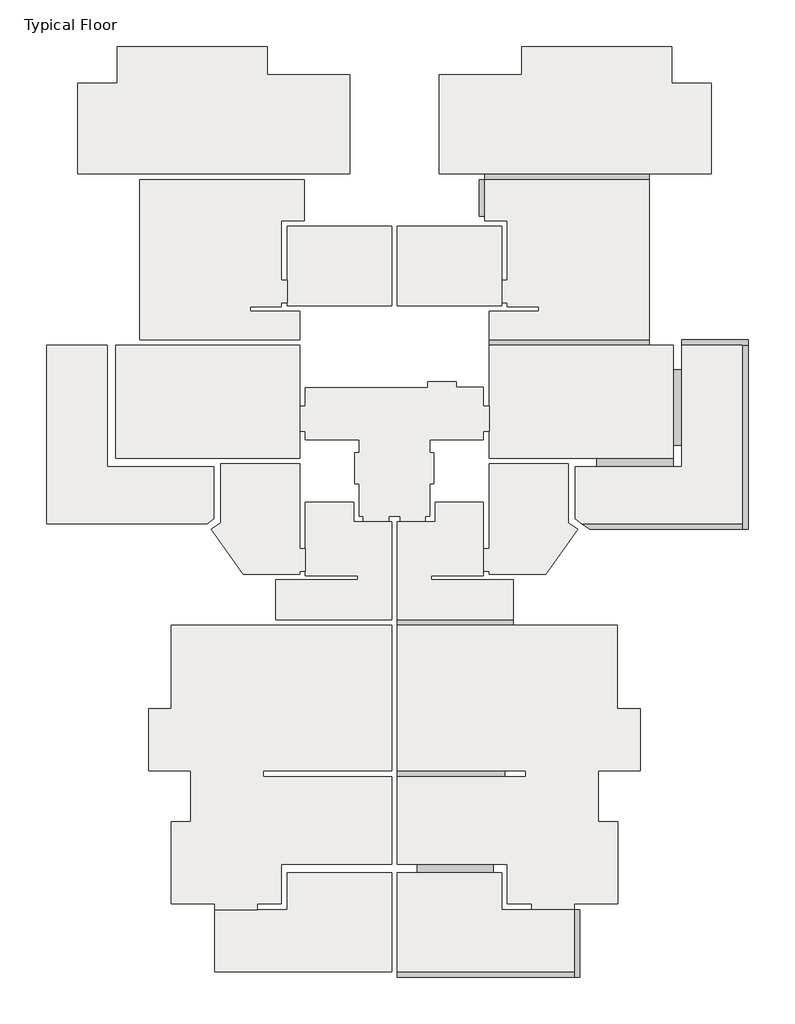
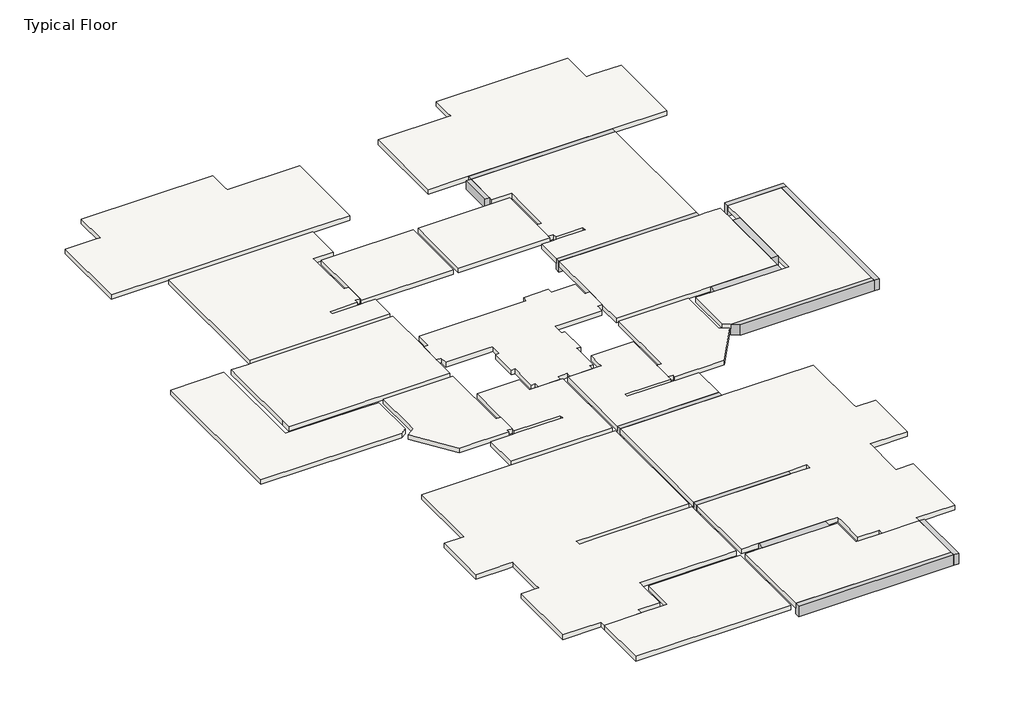
# One storey: 19 slabs, 13 beams.
"""IFC4 building model written with IfcOpenShell, lengths in millimetres."""

import ifcopenshell
import ifcopenshell.guid

model = None  # the IFC model being written
_history = None  # IfcOwnerHistory: only IFC2X3 demands one
_inside = {}  # id of a spatial element -> (the spatial element, [elements in it])
_under = {}  # id of a project, library or spatial element -> (it, [spatial elements below it])
_declared = {}  # id of a project -> (the project, [libraries it declares])
_typed = {}  # id of a type object -> (the type object, [elements of that type])
_made_of = {}  # id of a material, layer set ... -> (it, [elements and type objects made of it])


def new_model(schema):
    """Start an empty IFC model of exactly this schema.

    Asked for "IFC4X3", IfcOpenShell would pick the latest addendum, in which some entities
    have other attributes; the version numbers below select the first issue.
    IFC2X3 requires an IfcOwnerHistory on every rooted entity: one is made here for all.
    """
    global model, _history
    if schema == "IFC4X3":
        model = ifcopenshell.file(schema_version=(4, 3, 0, 0))
    else:
        model = ifcopenshell.file(schema=schema)
    _inside.clear()
    _under.clear()
    _declared.clear()
    _typed.clear()
    _made_of.clear()
    _history = None
    if model.schema == "IFC2X3":
        org = make("IfcOrganization", Name="unknown")
        user = make(
            "IfcPersonAndOrganization",
            ThePerson=make("IfcPerson", FamilyName="unknown"),
            TheOrganization=org,
        )
        app = make(
            "IfcApplication",
            ApplicationDeveloper=org,
            Version="unknown",
            ApplicationFullName="unknown",
            ApplicationIdentifier="unknown",
        )
        _history = make(
            "IfcOwnerHistory",
            OwningUser=user,
            OwningApplication=app,
            ChangeAction="ADDED",
            CreationDate=0,
        )
    return model


def make(cls, **values):
    """One entity of the class cls with the attributes given. An attribute that is None is left unset."""
    return model.create_entity(
        cls, **{name: value for name, value in values.items() if value is not None}
    )


def rooted(cls, **values):
    """An entity with a GlobalId (a new one), such as an element, a storey or a relation."""
    return make(cls, GlobalId=ifcopenshell.guid.new(), OwnerHistory=_history, **values)


def si_unit(unit_type, name, prefix=None):
    """IfcSIUnit, for example si_unit("LENGTHUNIT", "METRE", prefix="MILLI")."""
    return make("IfcSIUnit", UnitType=unit_type, Prefix=prefix, Name=name)


def assignment(units):
    """IfcUnitAssignment: the units of a project."""
    return None if units is None else make("IfcUnitAssignment", Units=units)


def point(xyz):
    """IfcCartesianPoint."""
    return None if xyz is None else make("IfcCartesianPoint", Coordinates=xyz)


def direction(xyz):
    """IfcDirection."""
    return None if xyz is None else make("IfcDirection", DirectionRatios=xyz)


def frame(location, z_axis=None, x_axis=None):
    """IfcAxis2Placement3D, a coordinate frame: its origin and axes. An axis left out is left unset."""
    return make(
        "IfcAxis2Placement3D",
        Location=point(location),
        Axis=direction(z_axis),
        RefDirection=direction(x_axis),
    )


def origin():
    """The frame at (0, 0, 0) with its axes left unset."""
    return frame((0.0, 0.0, 0.0))


def place(relative_to, where):
    """IfcLocalPlacement: puts the frame where relative to a parent placement (None: the world)."""
    return make(
        "IfcLocalPlacement", PlacementRelTo=relative_to, RelativePlacement=where
    )


def context(
    kind, dimensions, precision=None, world=None, true_north=None, identifier=None
):
    """IfcGeometricRepresentationContext, for example the 3D "Model" context."""
    return make(
        "IfcGeometricRepresentationContext",
        ContextIdentifier=identifier,
        ContextType=kind,
        CoordinateSpaceDimension=dimensions,
        Precision=precision,
        WorldCoordinateSystem=world,
        TrueNorth=true_north,
    )


def project(units=None, contexts=None):
    """IfcProject with its units and contexts."""
    return rooted(
        "IfcProject",
        Name="project",
        RepresentationContexts=contexts,
        UnitsInContext=assignment(units),
    )


def spatial(cls, under=None, at=None, **own):
    """A site, building, storey or space (cls), placed at a placement, below another one or the project."""
    s = rooted(cls, ObjectPlacement=at, **own)
    if under is not None:
        _under.setdefault(under.id(), (under, []))[1].append(s)
    return s


def faces_of(points, faces, orient=None, outer=None):
    """IfcFace entities. A face is a list of loops; a loop is a list of indices into points, from 0.

    orient and outer hold one flag for each loop. By default every Orientation is true, the
    first loop of a face is its IfcFaceOuterBound and the others are IfcFaceBound.
    """
    made = []
    for i, loops in enumerate(faces):
        bounds = []
        for j, loop in enumerate(loops):
            is_outer = j == 0 if outer is None else outer[i][j]
            bounds.append(
                make(
                    "IfcFaceOuterBound" if is_outer else "IfcFaceBound",
                    Bound=make("IfcPolyLoop", Polygon=[points[k] for k in loop]),
                    Orientation=True if orient is None else orient[i][j],
                )
            )
        made.append(make("IfcFace", Bounds=bounds))
    return made


def faceted_brep(points, faces, orient=None, outer=None, voids=None):
    """IfcFacetedBrep: a solid bounded by flat faces; with voids (closed shells), ...WithVoids."""
    shared = [point(p) for p in points]
    hull = make("IfcClosedShell", CfsFaces=faces_of(shared, faces, orient, outer))
    if voids is None:
        return make("IfcFacetedBrep", Outer=hull)
    return make(
        "IfcFacetedBrepWithVoids",
        Outer=hull,
        Voids=[
            make(cls, CfsFaces=faces_of(shared, fs, o, b)) for cls, fs, o, b in voids
        ],
    )


def shape(context_of_items, identifier, shape_type, items):
    """IfcShapeRepresentation: the items that make up one representation, for example the "Body"."""
    return make(
        "IfcShapeRepresentation",
        ContextOfItems=context_of_items,
        RepresentationIdentifier=identifier,
        RepresentationType=shape_type,
        Items=items,
    )


def made_of(thing, what):
    """Note that an element or type object is made of a material, layer set ...; save() writes the relation."""
    if what is not None:
        _made_of.setdefault(what.id(), (what, []))[1].append(thing)
    return thing


def element(
    cls,
    number,
    at=None,
    inside=None,
    cuts=None,
    type_object=None,
    material=None,
    context=None,
    identifier="Body",
    shape_type=None,
    held_by="IfcProductDefinitionShape",
    body=None,
    shapes=None,
    **own,
):
    """One element of the class cls, such as IfcWall. Its Tag is "e" and its number.

    at: its placement. inside: the storey or other place that contains it. cuts: it is an
    opening in that element (IfcRelVoidsElement). A single representation is given by context,
    identifier, shape_type and body (its items); several are given by shapes. held_by: the class
    of the entity that holds the representations. save() writes the other relations.
    """
    e = rooted(cls, Tag="e%d" % number, ObjectPlacement=at, **own)
    if body is not None:
        shapes = [shape(context, identifier, shape_type, body)]
    if shapes is not None:
        e.Representation = make(held_by, Representations=shapes)
    if inside is not None:
        _inside.setdefault(inside.id(), (inside, []))[1].append(e)
    if cuts is not None:
        rooted(
            "IfcRelVoidsElement", RelatingBuildingElement=cuts, RelatedOpeningElement=e
        )
    if type_object is not None:
        _typed.setdefault(type_object.id(), (type_object, []))[1].append(e)
    return made_of(e, material)


def aggregate(whole, parts):
    """IfcRelAggregates: a whole, such as a stair, and the parts it consists of."""
    return rooted("IfcRelAggregates", RelatingObject=whole, RelatedObjects=parts)


def save(model, path):
    """Write the relations noted so far, then the file.

    IfcRelAggregates (storeys below a building ...), IfcRelContainedInSpatialStructure (elements
    in a storey), IfcRelDefinesByType, IfcRelAssociatesMaterial and IfcRelDeclares: one each for
    every whole, place, type object, material and project.
    """
    for whole, parts in _under.values():
        aggregate(whole, parts)
    for where, things in _inside.values():
        rooted(
            "IfcRelContainedInSpatialStructure",
            RelatedElements=things,
            RelatingStructure=where,
        )
    for kind, things in _typed.values():
        rooted("IfcRelDefinesByType", RelatedObjects=things, RelatingType=kind)
    for what, things in _made_of.values():
        rooted("IfcRelAssociatesMaterial", RelatedObjects=things, RelatingMaterial=what)
    for by, libraries in _declared.values():
        rooted("IfcRelDeclares", RelatingContext=by, RelatedDefinitions=libraries)
    model.write(path)


model = new_model("IFC4")

# Units and contexts
model_context = context("Model", 3, world=origin())
ifc_project = project(units=[si_unit("LENGTHUNIT", "METRE", prefix="MILLI")], contexts=[model_context])

# Site, building, storey
site = spatial("IfcSite", under=ifc_project)
building = spatial("IfcBuilding", under=site)
storey = spatial("IfcBuildingStorey", under=building, Name="Typical Floor", Elevation=3000.0)

# Beams
placement = place(None, origin())
element("IfcBeam", 1, ObjectType="Concrete Rectengular Beam : 20/35", at=placement, inside=storey, context=model_context, shape_type="Brep", body=[
    faceted_brep([(7220.2839923, 5707.9881624, 3000.0), (7020.2839923, 5707.9881624, 3000.0), (7020.2839923, 4410.637169, 3000.0), (7220.2839923, 4410.637169, 3000.0), (7220.2839923, 5707.9881624, 2650.0), (7220.2839923, 5707.9881624, 2800.0), (7220.2839923, 4410.637169, 2650.0), (7020.2839923, 5707.9881624, 2650.0), (7020.2839923, 4410.637169, 2650.0)], [[[0, 1, 2, 3]], [[4, 5, 0, 3, 6]], [[7, 4, 6, 8]], [[1, 7, 8, 2]], [[1, 0, 5, 4, 7]], [[3, 2, 8, 6]]]),
])
element("IfcBeam", 2, ObjectType="Concrete Rectengular Beam : 20/45", at=placement, inside=storey, context=model_context, shape_type="Brep", body=[
    faceted_brep([(13024.2575022, -153.3363409, 3000.0), (13024.2575022, 46.6636591, 3000.0), (7369.9528665, 46.6636591, 3000.0), (7369.9528665, -153.3363409, 3000.0), (13024.2575022, -153.3363409, 2550.0), (7369.9528665, -153.3363409, 2800.0), (7369.9528665, -153.3363409, 2550.0), (13024.2575022, 46.6636591, 2550.0), (7369.9528665, 46.6636591, 2550.0), (13024.2575022, 46.6636591, 2800.0), (7369.9528665, 46.6636591, 2800.0)], [[[0, 1, 2, 3]], [[4, 0, 3, 5, 6]], [[7, 4, 6, 8]], [[1, 9, 7, 8, 10, 2]], [[1, 0, 4, 7, 9]], [[3, 2, 10, 8, 6, 5]]]),
])
element("IfcBeam", 3, ObjectType="Concrete Rectengular Beam : 20/45", at=placement, inside=storey, context=model_context, shape_type="Brep", body=[
    faceted_brep([(16525.1499872, -153.3363409, 3000.0), (16525.1499872, 46.6636591, 3000.0), (14175.1499872, 46.6636591, 3000.0), (14175.1499872, -153.3363409, 3000.0), (16325.1499872, -153.3363409, 3000.0), (16525.1499872, 46.6636591, 2550.0), (14175.1499872, 46.6636591, 2550.0), (16525.1499872, -153.3363409, 2550.0), (16325.1499872, -153.3363409, 2550.0), (14175.1499872, -153.3363409, 2550.0), (14175.1499872, -153.3363409, 2800.0)], [[[0, 1, 2, 3, 4]], [[1, 5, 6, 2]], [[5, 7, 8, 9, 6]], [[7, 0, 4, 3, 10, 9, 8]], [[3, 2, 6, 9, 10]], [[1, 0, 7, 5]]]),
])
element("IfcBeam", 4, ObjectType="Concrete Rectengular Beam : 20/45", at=placement, inside=storey, context=model_context, shape_type="Brep", body=[
    faceted_brep([(16325.1499872, -6653.3363409, 3000.0), (16525.1499872, -6653.3363409, 3000.0), (16525.1499872, -153.3363409, 3000.0), (16325.1499872, -153.3363409, 3000.0), (16325.1499872, -6453.3363409, 3000.0), (16525.1499872, -6653.3363409, 2550.0), (16525.1499872, -153.3363409, 2550.0), (16325.1499872, -6653.3363409, 2550.0), (16325.1499872, -6453.3363409, 2550.0), (16325.1499872, -153.3363409, 2550.0), (16325.1499872, -153.3363409, 2800.0)], [[[0, 1, 2, 3, 4]], [[1, 5, 6, 2]], [[5, 7, 8, 9, 6]], [[7, 0, 4, 3, 10, 9, 8]], [[3, 2, 6, 9, 10]], [[1, 0, 7, 5]]]),
])
element("IfcBeam", 5, ObjectType="Concrete Rectengular Beam : 20/45", at=placement, inside=storey, context=model_context, shape_type="Brep", body=[
    faceted_brep([(10651.3091706, -6453.3363409, 3000.0), (10931.7636873, -6652.8905163, 3000.0), (10931.4469171, -6653.3363409, 3000.0), (16325.1499872, -6653.3363409, 3000.0), (16325.1499872, -6453.3363409, 3000.0), (10931.4469171, -6653.3363409, 2550.0), (16325.1499872, -6653.3363409, 2550.0), (10931.7636873, -6652.8905163, 2550.0), (10651.3091706, -6453.3363409, 2550.0), (16325.1499872, -6453.3363409, 2550.0), (10651.3091706, -6453.3363409, 2800.0), (16325.1499872, -6453.3363409, 2800.0)], [[[0, 1, 2, 3, 4]], [[2, 5, 6, 3]], [[7, 8, 9, 6, 5]], [[8, 10, 0, 4, 11, 9]], [[1, 0, 10, 8, 7]], [[2, 1, 7, 5]], [[4, 3, 6, 9, 11]]]),
])
element("IfcBeam", 6, ObjectType="Concrete Rectengular Beam : 20/45", at=placement, inside=storey, context=model_context, shape_type="Brep", body=[
    faceted_brep([(10372.2707473, -22500.6211091, 3000.0), (10572.2707473, -22500.6211091, 3000.0), (10572.2707473, -20100.6211091, 3000.0), (10372.2707473, -20100.6211091, 3000.0), (10372.2707473, -22300.6211091, 3000.0), (10572.2707473, -22500.6211091, 2550.0), (10572.2707473, -20100.6211091, 2550.0), (10372.2707473, -22500.6211091, 2550.0), (10372.2707473, -22300.6211091, 2550.0), (10372.2707473, -20100.6211091, 2550.0), (10372.2707473, -20100.6211091, 2800.0)], [[[0, 1, 2, 3, 4]], [[1, 5, 6, 2]], [[5, 7, 8, 9, 6]], [[7, 0, 4, 3, 10, 9, 8]], [[3, 2, 6, 9, 10]], [[1, 0, 7, 5]]]),
])
element("IfcBeam", 7, ObjectType="Concrete Rectengular Beam : 20/45", at=placement, inside=storey, context=model_context, shape_type="Brep", body=[
    faceted_brep([(10372.2707473, -22500.6211091, 3000.0), (10372.2707473, -22300.6211091, 3000.0), (4123.5952506, -22300.6211091, 3000.0), (4123.5952506, -22500.6211091, 3000.0), (10372.2707473, -22500.6211091, 2550.0), (4123.5952506, -22500.6211091, 2550.0), (10372.2707473, -22300.6211091, 2550.0), (4123.5952506, -22300.6211091, 2550.0), (10372.2707473, -22300.6211091, 2800.0), (4123.5952506, -22300.6211091, 2800.0)], [[[0, 1, 2, 3]], [[4, 0, 3, 5]], [[6, 4, 5, 7]], [[1, 8, 6, 7, 9, 2]], [[1, 0, 4, 6, 8]], [[3, 2, 9, 7, 5]]]),
])
element("IfcBeam", 8, ObjectType="Concrete Rectengular Beam : 20/45", at=placement, inside=storey, context=model_context, shape_type="Brep", body=[
    faceted_brep([(7917.6091941, -15399.2157792, 3000.0), (7917.6091941, -15199.2157792, 3000.0), (4123.5952506, -15199.2157792, 3000.0), (4123.5952506, -15399.2157792, 3000.0), (7917.6091941, -15399.2157792, 2550.0), (7917.6091941, -15399.2157792, 2800.0), (4123.5952506, -15399.2157792, 2800.0), (4123.5952506, -15399.2157792, 2550.0), (7917.6091941, -15199.2157792, 2550.0), (4123.5952506, -15199.2157792, 2550.0), (7917.6091941, -15199.2157792, 2800.0), (4123.5952506, -15199.2157792, 2800.0)], [[[0, 1, 2, 3]], [[4, 5, 0, 3, 6, 7]], [[8, 4, 7, 9]], [[1, 10, 8, 9, 11, 2]], [[1, 0, 5, 4, 8, 10]], [[3, 2, 11, 9, 7, 6]]]),
])
element("IfcBeam", 9, ObjectType="Concrete Rectengular Beam : 20/45", at=placement, inside=storey, context=model_context, shape_type="Brep", body=[
    faceted_brep([(8220.6151181, -10045.6542217, 3000.0), (8220.6151181, -9845.6542217, 3000.0), (4123.5952506, -9845.6542217, 3000.0), (4123.5952506, -10045.6542217, 3000.0), (8220.6151181, -10045.6542217, 2550.0), (4123.5952506, -10045.6542217, 2800.0), (4123.5952506, -10045.6542217, 2550.0), (8220.6151181, -9845.6542217, 2550.0), (4123.5952506, -9845.6542217, 2550.0), (8220.6151181, -9845.6542217, 2800.0), (4123.5952506, -9845.6542217, 2800.0)], [[[0, 1, 2, 3]], [[4, 0, 3, 5, 6]], [[7, 4, 6, 8]], [[1, 9, 7, 8, 10, 2]], [[1, 0, 4, 7, 9]], [[3, 2, 10, 8, 6, 5]]]),
])
element("IfcBeam", 10, ObjectType="Concrete Rectengular Beam : 20/45", at=placement, inside=storey, context=model_context, shape_type="Brep", body=[
    faceted_brep([(13024.2575022, 5707.9881624, 3000.0), (13024.2575022, 5907.9881624, 3000.0), (7220.2839923, 5907.9881624, 3000.0), (7220.2839923, 5707.9881624, 3000.0), (13024.2575022, 5707.9881624, 2550.0), (13024.2575022, 5707.9881624, 2800.0), (7220.2839923, 5707.9881624, 2800.0), (7220.2839923, 5707.9881624, 2550.0), (13024.2575022, 5907.9881624, 2550.0), (7220.2839923, 5907.9881624, 2550.0)], [[[0, 1, 2, 3]], [[4, 5, 0, 3, 6, 7]], [[8, 4, 7, 9]], [[1, 8, 9, 2]], [[1, 0, 5, 4, 8]], [[3, 2, 9, 7, 6]]]),
])
element("IfcBeam", 11, ObjectType="Concrete Rectengular Beam : 30/45", at=placement, inside=storey, context=model_context, shape_type="Brep", body=[
    faceted_brep([(7522.2707473, -18796.3164734, 3000.0), (7522.2707473, -18496.3164734, 3000.0), (4828.2310122, -18496.3164734, 3000.0), (4828.2310122, -18796.3164734, 3000.0), (7522.2707473, -18496.3164734, 2800.0), (7522.2707473, -18496.3164734, 2550.0), (4828.2310122, -18496.3164734, 2550.0), (7522.2707473, -18796.3164734, 2550.0), (4828.2310122, -18796.3164734, 2550.0)], [[[0, 1, 2, 3]], [[1, 4, 5, 6, 2]], [[5, 7, 8, 6]], [[7, 0, 3, 8]], [[1, 0, 7, 5, 4]], [[3, 2, 6, 8]]]),
])
element("IfcBeam", 12, ObjectType="Concrete Rectengular Beam : 30/45", at=placement, inside=storey, context=model_context, shape_type="Brep", body=[
    faceted_brep([(13874.4026477, -4440.6873343, 3000.0), (13874.4026477, -4140.6873343, 3000.0), (11177.9817051, -4140.6873343, 3000.0), (11177.9817051, -4440.6873343, 3000.0), (13874.4026477, -4140.6873343, 2800.0), (13874.4026477, -4140.6873343, 2550.0), (11177.9817051, -4140.6873343, 2550.0), (13874.4026477, -4440.6873343, 2550.0), (11177.9817051, -4440.6873343, 2550.0), (11177.9817051, -4440.6873343, 2800.0), (13874.4026477, -4440.6873343, 2800.0)], [[[0, 1, 2, 3]], [[1, 4, 5, 6, 2]], [[5, 7, 8, 6]], [[0, 3, 9, 8, 7, 10]], [[1, 0, 10, 7, 5, 4]], [[3, 2, 6, 8, 9]]]),
])
element("IfcBeam", 13, ObjectType="Concrete Rectengular Beam : 30/45", at=placement, inside=storey, context=model_context, shape_type="Brep", body=[
    faceted_brep([(13875.1499872, -770.4005958, 2550.0), (13874.4026477, -770.4005958, 2550.0), (13874.4026477, -770.4005958, 2800.0), (13875.1499872, -770.4005958, 2800.0), (14174.4026477, -1013.3363409, 3000.0), (13875.1499872, -1013.3363409, 3000.0), (13875.1499872, -3690.6873343, 3000.0), (14174.4026477, -3690.6873343, 3000.0), (13874.4026477, -3690.6873343, 2550.0), (13874.4026477, -3690.6873343, 2800.0), (13875.1499872, -1013.3363409, 2550.0), (14174.4026477, -1013.3363409, 2550.0), (14174.4026477, -3690.6873343, 2550.0), (14174.4026477, -3690.6873343, 2800.0), (14174.4026477, -1013.3363409, 2800.0), (13875.1499872, -3690.6873343, 2800.0), (13875.1499872, -1013.3363409, 2800.0)], [[[0, 1, 2, 3]], [[4, 5, 6, 7]], [[1, 8, 9, 2]], [[8, 1, 0, 10, 11, 12]], [[4, 7, 13, 12, 11, 14]], [[8, 12, 13, 7, 6, 15, 9]], [[5, 4, 14, 11, 10, 16]], [[3, 2, 9, 15, 16]], [[6, 5, 16, 15]], [[10, 0, 3, 16]]]),
])

# Slabs
element("IfcSlab", 14, ObjectType="20", at=placement, inside=storey, context=model_context, shape_type="Brep", body=[
    faceted_brep([(-5775.4113719, 9110.3060432, 2800.0), (-5775.4113719, 10413.9484273, 2800.0), (-475.4113719, 10413.9484273, 2800.0), (-475.4113719, 9607.9881624, 2800.0), (-475.4113719, 9407.9881624, 2800.0), (2439.2609277, 9407.9881624, 2800.0), (2439.2609277, 5907.9881624, 2800.0), (-7177.0670011, 5907.9881624, 2800.0), (-7177.0670011, 9110.3060432, 2800.0), (-5975.4113719, 9110.3060432, 2800.0), (-5775.4113719, 10413.9484273, 3000.0), (-5775.4113719, 9110.3060432, 3000.0), (-5975.4113719, 9110.3060432, 3000.0), (-7177.0670011, 9110.3060432, 3000.0), (-7177.0670011, 5907.9881624, 3000.0), (-4977.0670011, 5907.9881624, 3000.0), (826.9065089, 5907.9881624, 3000.0), (2439.2609277, 5907.9881624, 3000.0), (2439.2609277, 9407.9881624, 3000.0), (-475.4113719, 9407.9881624, 3000.0), (-475.4113719, 9607.9881624, 3000.0), (-475.4113719, 10413.9484273, 3000.0)], [[[0, 1, 2, 3, 4, 5, 6, 7, 8, 9]], [[10, 11, 12, 13, 14, 15, 16, 17, 18, 19, 20, 21]], [[11, 0, 9, 8, 13, 12]], [[1, 0, 11, 10]], [[2, 1, 10, 21]], [[2, 21, 20, 19, 4, 3]], [[5, 4, 19, 18]], [[6, 5, 18, 17]], [[7, 6, 17, 16, 15, 14]], [[8, 7, 14, 13]]]),
])
element("IfcSlab", 15, ObjectType="20", at=placement, inside=storey, context=model_context, shape_type="Brep", body=[
    faceted_brep([(-4977.0670011, 5707.9881624, 2800.0), (826.9065089, 5707.9881624, 2800.0), (826.9065089, 4260.637169, 2800.0), (27.8998864, 4260.637169, 2800.0), (27.8998864, 4060.637169, 2800.0), (27.8998864, 2158.3192882, 2800.0), (227.8998864, 2158.3192882, 2800.0), (227.8998864, 1353.021275, 2800.0), (27.8998864, 1353.021275, 2800.0), (27.8998864, 1207.3259107, 2800.0), (-1073.0934911, 1207.3259107, 2800.0), (-1073.0934911, 1057.3259107, 2800.0), (27.8998864, 1057.3259107, 2800.0), (227.8998864, 1057.3259107, 2800.0), (675.9131314, 1057.3259107, 2800.0), (675.9131314, 46.6636591, 2800.0), (-4977.0670011, 46.6636591, 2800.0), (826.9065089, 5707.9881624, 3000.0), (-4977.0670011, 5707.9881624, 3000.0), (-4977.0670011, 46.6636591, 3000.0), (675.9131314, 46.6636591, 3000.0), (675.9131314, 1057.3259107, 3000.0), (227.8998864, 1057.3259107, 3000.0), (27.8998864, 1057.3259107, 3000.0), (-1073.0934911, 1057.3259107, 3000.0), (-1073.0934911, 1207.3259107, 3000.0), (27.8998864, 1207.3259107, 3000.0), (27.8998864, 1353.021275, 3000.0), (227.8998864, 1353.021275, 3000.0), (227.8998864, 2158.3192882, 3000.0), (27.8998864, 2158.3192882, 3000.0), (27.8998864, 4060.637169, 3000.0), (27.8998864, 4260.637169, 3000.0), (826.9065089, 4260.637169, 3000.0), (826.9065089, 4410.637169, 3000.0)], [[[0, 1, 2, 3, 4, 5, 6, 7, 8, 9, 10, 11, 12, 13, 14, 15, 16]], [[17, 18, 19, 20, 21, 22, 23, 24, 25, 26, 27, 28, 29, 30, 31, 32, 33, 34]], [[1, 0, 18, 17]], [[2, 1, 17, 34, 33]], [[3, 2, 33, 32]], [[3, 32, 31, 30, 5, 4]], [[6, 5, 30, 29]], [[7, 6, 29, 28]], [[8, 7, 28, 27]], [[9, 8, 27, 26]], [[10, 9, 26, 25]], [[11, 10, 25, 24]], [[11, 24, 23, 22, 21, 14, 13, 12]], [[15, 14, 21, 20]], [[16, 15, 20, 19]], [[0, 16, 19, 18]]]),
])
element("IfcSlab", 16, ObjectType="20", at=placement, inside=storey, context=model_context, shape_type="Brep", body=[
    faceted_brep([(3928.562138, 1257.3259107, 2800.0), (227.8998864, 1257.3259107, 2800.0), (227.8998864, 1353.021275, 2800.0), (227.8998864, 2158.3192882, 2800.0), (227.8998864, 4060.637169, 2800.0), (3928.562138, 4060.637169, 2800.0), (227.8998864, 1257.3259107, 3000.0), (3928.562138, 1257.3259107, 3000.0), (3928.562138, 4060.637169, 3000.0), (826.9065089, 4060.637169, 3000.0), (227.8998864, 4060.637169, 3000.0), (227.8998864, 2158.3192882, 3000.0), (227.8998864, 1353.021275, 3000.0)], [[[0, 1, 2, 3, 4, 5]], [[6, 7, 8, 9, 10, 11, 12]], [[7, 0, 5, 8]], [[1, 0, 7, 6]], [[1, 6, 12, 11, 10, 4, 3, 2]], [[4, 10, 9, 8, 5]]]),
])
element("IfcSlab", 17, ObjectType="20", at=placement, inside=storey, context=model_context, shape_type="Brep", body=[
    faceted_brep([(675.9131314, -153.3363409, 2800.0), (675.9131314, -2295.9853475, 2800.0), (675.9131314, -3195.6542217, 2800.0), (675.9131314, -4140.6873343, 2800.0), (-5827.2121465, -4140.6873343, 2800.0), (-5827.2121465, -3690.6873343, 2800.0), (-5827.9594861, -3690.6873343, 2800.0), (-5827.9594861, -1013.3363409, 2800.0), (-5827.9594861, -770.4005958, 2800.0), (-5827.9594861, -153.3363409, 2800.0), (675.9131314, -4140.6873343, 3000.0), (675.9131314, -3195.6542217, 3000.0), (675.9131314, -2295.9853475, 3000.0), (675.9131314, -153.3363409, 3000.0), (-4977.0670011, -153.3363409, 3000.0), (-5177.0670011, -153.3363409, 3000.0), (-5827.9594861, -153.3363409, 3000.0), (-5827.9594861, -1013.3363409, 3000.0), (-5827.9594861, -3690.6873343, 3000.0), (-5827.2121465, -3690.6873343, 3000.0), (-5827.2121465, -4140.6873343, 3000.0), (-3130.7912039, -4140.6873343, 3000.0), (-2370.7912039, -4140.6873343, 3000.0), (-2120.7912039, -4140.6873343, 3000.0)], [[[0, 1, 2, 3, 4, 5, 6, 7, 8, 9]], [[10, 11, 12, 13, 14, 15, 16, 17, 18, 19, 20, 21, 22, 23]], [[3, 2, 1, 0, 13, 12, 11, 10]], [[3, 10, 23, 22, 21, 20, 4]], [[16, 9, 8, 7, 6, 18, 17]], [[0, 9, 16, 15, 14, 13]], [[19, 5, 4, 20]], [[5, 19, 18, 6]]]),
])
element("IfcSlab", 18, ObjectType="20", at=placement, inside=storey, context=model_context, shape_type="Brep", body=[
    faceted_brep([(-8277.9594861, -6453.3363409, 2800.0), (-8277.9594861, -153.3363409, 2800.0), (-6127.9594861, -153.3363409, 2800.0), (-6127.9594861, -1013.3363409, 2800.0), (-6127.2121465, -1013.3363409, 2800.0), (-6127.2121465, -3690.6873343, 2800.0), (-6127.2121465, -4440.6873343, 2800.0), (-5827.2121465, -4440.6873343, 2800.0), (-3130.7912039, -4440.6873343, 2800.0), (-2370.7912039, -4440.6873343, 2800.0), (-2370.7912039, -6287.3148751, 2800.0), (-2604.1186694, -6453.3363409, 2800.0), (-8277.9594861, -153.3363409, 3000.0), (-8277.9594861, -6453.3363409, 3000.0), (-2604.1186694, -6453.3363409, 3000.0), (-2370.7912039, -6287.3148751, 3000.0), (-2370.7912039, -4440.6873343, 3000.0), (-3130.7912039, -4440.6873343, 3000.0), (-5827.2121465, -4440.6873343, 3000.0), (-6127.2121465, -4440.6873343, 3000.0), (-6127.2121465, -3690.6873343, 3000.0), (-6127.2121465, -1013.3363409, 3000.0), (-6127.9594861, -1013.3363409, 3000.0), (-6127.9594861, -153.3363409, 3000.0)], [[[0, 1, 2, 3, 4, 5, 6, 7, 8, 9, 10, 11]], [[12, 13, 14, 15, 16, 17, 18, 19, 20, 21, 22, 23]], [[1, 12, 23, 2]], [[19, 6, 5, 4, 21, 20]], [[6, 19, 18, 17, 16, 9, 8, 7]], [[9, 16, 15, 10]], [[13, 0, 11, 14]], [[1, 0, 13, 12]], [[22, 3, 2, 23]], [[3, 22, 21, 4]], [[11, 10, 15, 14]]]),
])
element("IfcSlab", 19, ObjectType="20", at=placement, inside=storey, context=model_context, shape_type="Brep", body=[
    faceted_brep([(675.9131314, -4340.6873343, 2800.0), (675.9131314, -7341.6807118, 2800.0), (875.9131314, -7341.6807118, 2800.0), (877.2376347, -7341.6807118, 2800.0), (877.2376347, -8146.978725, 2800.0), (677.2376347, -8146.978725, 2800.0), (677.2376347, -8247.6409767, 2800.0), (-1322.1082056, -8247.6409767, 2800.0), (-2454.5945115, -6653.7713609, 2800.0), (-2120.7912039, -6416.257469, 2800.0), (-2120.7912039, -6109.4302597, 2800.0), (-2120.7912039, -4340.6873343, 2800.0), (675.9131314, -7341.6807118, 3000.0), (675.9131314, -4340.6873343, 3000.0), (-2120.7912039, -4340.6873343, 3000.0), (-2120.7912039, -6109.4302597, 3000.0), (-2120.7912039, -6416.257469, 3000.0), (-2454.5945115, -6653.7713609, 3000.0), (-1322.1082056, -8247.6409767, 3000.0), (-373.424617, -8247.6409767, 3000.0), (-173.424617, -8247.6409767, 3000.0), (677.2376347, -8247.6409767, 3000.0), (677.2376347, -8146.978725, 3000.0), (877.2376347, -8146.978725, 3000.0), (877.2376347, -7341.6807118, 3000.0), (875.9131314, -7341.6807118, 3000.0)], [[[0, 1, 2, 3, 4, 5, 6, 7, 8, 9, 10, 11]], [[12, 13, 14, 15, 16, 17, 18, 19, 20, 21, 22, 23, 24, 25]], [[1, 0, 13, 12]], [[1, 12, 25, 24, 3, 2]], [[4, 3, 24, 23]], [[5, 4, 23, 22]], [[6, 5, 22, 21]], [[6, 21, 20, 19, 18, 7]], [[16, 9, 8, 17]], [[9, 16, 15, 14, 11, 10]], [[0, 11, 14, 13]], [[8, 7, 18, 17]]]),
])
element("IfcSlab", 20, ObjectType="20", at=placement, inside=storey, context=model_context, shape_type="Brep", body=[
    faceted_brep([(875.9131314, -5693.3363409, 2800.0), (2577.2376347, -5693.3363409, 2800.0), (2577.2376347, -6191.6807118, 2800.0), (2577.2376347, -6391.6807118, 2800.0), (2928.2310122, -6391.6807118, 2800.0), (3827.8998864, -6391.6807118, 2800.0), (3923.5952506, -6391.6807118, 2800.0), (3923.5952506, -9845.6542217, 2800.0), (-173.424617, -9845.6542217, 2800.0), (-173.424617, -8447.6409767, 2800.0), (677.2376347, -8447.6409767, 2800.0), (877.2376347, -8447.6409767, 2800.0), (2726.9065089, -8447.6409767, 2800.0), (2726.9065089, -8297.6409767, 2800.0), (877.2376347, -8297.6409767, 2800.0), (877.2376347, -8146.978725, 2800.0), (877.2376347, -7341.6807118, 2800.0), (875.9131314, -7341.6807118, 2800.0), (2577.2376347, -5693.3363409, 3000.0), (875.9131314, -5693.3363409, 3000.0), (875.9131314, -7341.6807118, 3000.0), (877.2376347, -7341.6807118, 3000.0), (877.2376347, -8146.978725, 3000.0), (877.2376347, -8297.6409767, 3000.0), (2726.9065089, -8297.6409767, 3000.0), (2726.9065089, -8447.6409767, 3000.0), (877.2376347, -8447.6409767, 3000.0), (677.2376347, -8447.6409767, 3000.0), (-173.424617, -8447.6409767, 3000.0), (-173.424617, -9845.6542217, 3000.0), (3923.5952506, -9845.6542217, 3000.0), (3923.5952506, -6391.6807118, 3000.0), (3827.8998864, -6391.6807118, 3000.0), (2928.2310122, -6391.6807118, 3000.0), (2577.2376347, -6391.6807118, 3000.0), (2577.2376347, -6191.6807118, 3000.0)], [[[0, 1, 2, 3, 4, 5, 6, 7, 8, 9, 10, 11, 12, 13, 14, 15, 16, 17]], [[18, 19, 20, 21, 22, 23, 24, 25, 26, 27, 28, 29, 30, 31, 32, 33, 34, 35]], [[1, 0, 19, 18]], [[1, 18, 35, 34, 3, 2]], [[4, 3, 34, 33]], [[4, 33, 32, 31, 6, 5]], [[7, 6, 31, 30]], [[8, 7, 30, 29]], [[9, 8, 29, 28]], [[9, 28, 27, 26, 25, 12, 11, 10]], [[13, 12, 25, 24]], [[13, 24, 23, 14]], [[19, 0, 17, 20]], [[14, 23, 22, 21, 16, 15]], [[16, 21, 20, 17]]]),
])
element("IfcSlab", 21, ObjectType="20", at=placement, inside=storey, context=model_context, shape_type="Brep", body=[
    faceted_brep([(3923.5952506, -10045.6542217, 2800.0), (3923.5952506, -15199.2157792, 2800.0), (129.5813071, -15199.2157792, 2800.0), (-620.4186929, -15199.2157792, 2800.0), (-620.4186929, -15399.2157792, 2800.0), (129.5813071, -15399.2157792, 2800.0), (3923.5952506, -15399.2157792, 2800.0), (3923.5952506, -18496.3164734, 2800.0), (3223.9263764, -18496.3164734, 2800.0), (524.9197539, -18496.3164734, 2800.0), (27.8998864, -18496.3164734, 2800.0), (27.8998864, -18796.3164734, 2800.0), (27.8998864, -19900.6211091, 2800.0), (-827.7292527, -19900.6211091, 2800.0), (-827.7292527, -20100.6211091, 2800.0), (-2325.0802461, -20100.6211091, 2800.0), (-2325.0802461, -19900.6211091, 2800.0), (-3874.0868686, -19900.6211091, 2800.0), (-3874.0868686, -16998.96548, 2800.0), (-3174.4179944, -16998.96548, 2800.0), (-3174.4179944, -16798.96548, 2800.0), (-3174.4179944, -15196.978725, 2800.0), (-3374.4179944, -15196.978725, 2800.0), (-4673.0934911, -15196.978725, 2800.0), (-4673.0934911, -12996.3164734, 2800.0), (-3860.1795838, -12996.3164734, 2800.0), (-3860.1795838, -12796.3164734, 2800.0), (-3860.1795838, -10045.6542217, 2800.0), (3923.5952506, -15199.2157792, 3000.0), (3923.5952506, -10045.6542217, 3000.0), (-173.424617, -10045.6542217, 3000.0), (-3860.1795838, -10045.6542217, 3000.0), (-3860.1795838, -12796.3164734, 3000.0), (-3860.1795838, -12996.3164734, 3000.0), (-4673.0934911, -12996.3164734, 3000.0), (-4673.0934911, -15196.978725, 3000.0), (-3374.4179944, -15196.978725, 3000.0), (-3174.4179944, -15196.978725, 3000.0), (-3174.4179944, -16798.96548, 3000.0), (-3174.4179944, -16998.96548, 3000.0), (-3874.0868686, -16998.96548, 3000.0), (-3874.0868686, -19900.6211091, 3000.0), (-2325.0802461, -19900.6211091, 3000.0), (-2325.0802461, -20100.6211091, 3000.0), (-827.7292527, -20100.6211091, 3000.0), (-827.7292527, -19900.6211091, 3000.0), (27.8998864, -19900.6211091, 3000.0), (27.8998864, -18796.3164734, 3000.0), (27.8998864, -18496.3164734, 3000.0), (524.9197539, -18496.3164734, 3000.0), (3223.9263764, -18496.3164734, 3000.0), (3923.5952506, -18496.3164734, 3000.0), (3923.5952506, -15399.2157792, 3000.0), (129.5813071, -15399.2157792, 3000.0), (-620.4186929, -15399.2157792, 3000.0), (-620.4186929, -15199.2157792, 3000.0), (129.5813071, -15199.2157792, 3000.0)], [[[0, 1, 2, 3, 4, 5, 6, 7, 8, 9, 10, 11, 12, 13, 14, 15, 16, 17, 18, 19, 20, 21, 22, 23, 24, 25, 26, 27]], [[28, 29, 30, 31, 32, 33, 34, 35, 36, 37, 38, 39, 40, 41, 42, 43, 44, 45, 46, 47, 48, 49, 50, 51, 52, 53, 54, 55, 56]], [[1, 0, 29, 28]], [[1, 28, 56, 55, 3, 2]], [[4, 3, 55, 54]], [[4, 54, 53, 52, 6, 5]], [[7, 6, 52, 51]], [[7, 51, 50, 49, 48, 10, 9, 8]], [[10, 48, 47, 46, 12, 11]], [[13, 12, 46, 45]], [[14, 13, 45, 44]], [[15, 14, 44, 43]], [[16, 15, 43, 42]], [[17, 16, 42, 41]], [[18, 17, 41, 40]], [[19, 18, 40, 39]], [[19, 39, 38, 37, 21, 20]], [[21, 37, 36, 35, 23, 22]], [[24, 23, 35, 34]], [[25, 24, 34, 33]], [[25, 33, 32, 31, 27, 26]], [[0, 27, 31, 30, 29]]]),
])
element("IfcSlab", 22, ObjectType="20", at=placement, inside=storey, context=model_context, shape_type="Brep", body=[
    faceted_brep([(227.8998864, -20100.6211091, 2800.0), (227.8998864, -18796.3164734, 2800.0), (3923.5952506, -18796.3164734, 2800.0), (3923.5952506, -22300.6211091, 2800.0), (-2325.0802461, -22300.6211091, 2800.0), (-2325.0802461, -20100.6211091, 2800.0), (-827.7292527, -20100.6211091, 2800.0), (27.8998864, -20100.6211091, 2800.0), (227.8998864, -18796.3164734, 3000.0), (227.8998864, -20100.6211091, 3000.0), (27.8998864, -20100.6211091, 3000.0), (-827.7292527, -20100.6211091, 3000.0), (-2325.0802461, -20100.6211091, 3000.0), (-2325.0802461, -22300.6211091, 3000.0), (3923.5952506, -22300.6211091, 3000.0), (3923.5952506, -18796.3164734, 3000.0), (3223.9263764, -18796.3164734, 3000.0), (524.9197539, -18796.3164734, 3000.0)], [[[0, 1, 2, 3, 4, 5, 6, 7]], [[8, 9, 10, 11, 12, 13, 14, 15, 16, 17]], [[1, 0, 9, 8]], [[2, 1, 8, 17, 16, 15]], [[3, 2, 15, 14]], [[4, 3, 14, 13]], [[5, 4, 13, 12]], [[5, 12, 11, 10, 9, 0, 7, 6]]]),
])
element("IfcSlab", 23, ObjectType="20", at=placement, inside=storey, context=model_context, shape_type="Brep", body=[
    faceted_brep([(13822.6018731, 10413.9484273, 2800.0), (13822.6018731, 9110.3060432, 2800.0), (14022.6018731, 9110.3060432, 2800.0), (15224.2575022, 9110.3060432, 2800.0), (15224.2575022, 5907.9881624, 2800.0), (5607.9295735, 5907.9881624, 2800.0), (5607.9295735, 9407.9881624, 2800.0), (8522.6018731, 9407.9881624, 2800.0), (8522.6018731, 9607.9881624, 2800.0), (8522.6018731, 10413.9484273, 2800.0), (13822.6018731, 9110.3060432, 3000.0), (13822.6018731, 10413.9484273, 3000.0), (8522.6018731, 10413.9484273, 3000.0), (8522.6018731, 9607.9881624, 3000.0), (8522.6018731, 9407.9881624, 3000.0), (5607.9295735, 9407.9881624, 3000.0), (5607.9295735, 5907.9881624, 3000.0), (7220.2839923, 5907.9881624, 3000.0), (13024.2575022, 5907.9881624, 3000.0), (15224.2575022, 5907.9881624, 3000.0), (15224.2575022, 9110.3060432, 3000.0), (14022.6018731, 9110.3060432, 3000.0)], [[[0, 1, 2, 3, 4, 5, 6, 7, 8, 9]], [[10, 11, 12, 13, 14, 15, 16, 17, 18, 19, 20, 21]], [[1, 10, 21, 20, 3, 2]], [[1, 0, 11, 10]], [[0, 9, 12, 11]], [[7, 14, 13, 12, 9, 8]], [[7, 6, 15, 14]], [[6, 5, 16, 15]], [[5, 4, 19, 18, 17, 16]], [[4, 3, 20, 19]]]),
])
element("IfcSlab", 24, ObjectType="20", at=placement, inside=storey, context=model_context, shape_type="Brep", body=[
    faceted_brep([(7220.2839923, 5707.9881624, 2800.0), (13024.2575022, 5707.9881624, 2800.0), (13024.2575022, 46.6636591, 2800.0), (7369.9528665, 46.6636591, 2800.0), (7369.9528665, 1057.3259107, 2800.0), (7819.2906148, 1057.3259107, 2800.0), (8019.2906148, 1057.3259107, 2800.0), (9120.2839923, 1057.3259107, 2800.0), (9120.2839923, 1207.3259107, 2800.0), (8019.2906148, 1207.3259107, 2800.0), (8019.2906148, 1353.021275, 2800.0), (7819.2906148, 1353.021275, 2800.0), (7819.2906148, 2158.3192882, 2800.0), (8019.2906148, 2158.3192882, 2800.0), (8019.2906148, 4060.637169, 2800.0), (8019.2906148, 4260.637169, 2800.0), (7220.2839923, 4260.637169, 2800.0), (13024.2575022, 5707.9881624, 3000.0), (7220.2839923, 5707.9881624, 3000.0), (7220.2839923, 4410.637169, 3000.0), (7220.2839923, 4260.637169, 3000.0), (8019.2906148, 4260.637169, 3000.0), (8019.2906148, 4060.637169, 3000.0), (8019.2906148, 2158.3192882, 3000.0), (7819.2906148, 2158.3192882, 3000.0), (7819.2906148, 1353.021275, 3000.0), (8019.2906148, 1353.021275, 3000.0), (8019.2906148, 1207.3259107, 3000.0), (9120.2839923, 1207.3259107, 3000.0), (9120.2839923, 1057.3259107, 3000.0), (8019.2906148, 1057.3259107, 3000.0), (7819.2906148, 1057.3259107, 3000.0), (7369.9528665, 1057.3259107, 3000.0), (7369.9528665, 46.6636591, 3000.0), (13024.2575022, 46.6636591, 3000.0)], [[[0, 1, 2, 3, 4, 5, 6, 7, 8, 9, 10, 11, 12, 13, 14, 15, 16]], [[17, 18, 19, 20, 21, 22, 23, 24, 25, 26, 27, 28, 29, 30, 31, 32, 33, 34]], [[1, 0, 18, 17]], [[0, 16, 20, 19, 18]], [[16, 15, 21, 20]], [[13, 23, 22, 21, 15, 14]], [[13, 12, 24, 23]], [[12, 11, 25, 24]], [[11, 10, 26, 25]], [[10, 9, 27, 26]], [[9, 8, 28, 27]], [[8, 7, 29, 28]], [[4, 32, 31, 30, 29, 7, 6, 5]], [[4, 3, 33, 32]], [[3, 2, 34, 33]], [[2, 1, 17, 34]]]),
])
element("IfcSlab", 25, ObjectType="20", at=placement, inside=storey, context=model_context, shape_type="Brep", body=[
    faceted_brep([(7819.2906148, 1257.3259107, 2800.0), (4128.562138, 1257.3259107, 2800.0), (4128.562138, 4060.637169, 2800.0), (7819.2906148, 4060.637169, 2800.0), (7819.2906148, 2158.3192882, 2800.0), (7819.2906148, 1353.021275, 2800.0), (4128.562138, 1257.3259107, 3000.0), (7819.2906148, 1257.3259107, 3000.0), (7819.2906148, 1353.021275, 3000.0), (7819.2906148, 2158.3192882, 3000.0), (7819.2906148, 4060.637169, 3000.0), (7220.2839923, 4060.637169, 3000.0), (4128.562138, 4060.637169, 3000.0)], [[[0, 1, 2, 3, 4, 5]], [[6, 7, 8, 9, 10, 11, 12]], [[1, 6, 12, 2]], [[1, 0, 7, 6]], [[7, 0, 5, 4, 3, 10, 9, 8]], [[2, 12, 11, 10, 3]]]),
])
element("IfcSlab", 26, ObjectType="20", at=placement, inside=storey, context=model_context, shape_type="Brep", body=[
    faceted_brep([(7369.9528665, -4140.6873343, 2800.0), (7369.9528665, -3195.6542217, 2800.0), (7369.9528665, -2295.9853475, 2800.0), (7369.9528665, -153.3363409, 2800.0), (13875.1499872, -153.3363409, 2800.0), (13875.1499872, -770.4005958, 2800.0), (13875.1499872, -1013.3363409, 2800.0), (13875.1499872, -3690.6873343, 2800.0), (13874.4026477, -3690.6873343, 2800.0), (13874.4026477, -4140.6873343, 2800.0), (7369.9528665, -153.3363409, 3000.0), (7369.9528665, -2295.9853475, 3000.0), (7369.9528665, -3195.6542217, 3000.0), (7369.9528665, -4140.6873343, 3000.0), (10167.9817051, -4140.6873343, 3000.0), (10417.9817051, -4140.6873343, 3000.0), (11177.9817051, -4140.6873343, 3000.0), (13874.4026477, -4140.6873343, 3000.0), (13874.4026477, -3690.6873343, 3000.0), (13875.1499872, -3690.6873343, 3000.0), (13875.1499872, -1013.3363409, 3000.0), (13875.1499872, -153.3363409, 3000.0), (13224.2575022, -153.3363409, 3000.0), (13024.2575022, -153.3363409, 3000.0)], [[[0, 1, 2, 3, 4, 5, 6, 7, 8, 9]], [[10, 11, 12, 13, 14, 15, 16, 17, 18, 19, 20, 21, 22, 23]], [[3, 2, 1, 0, 13, 12, 11, 10]], [[13, 0, 9, 17, 16, 15, 14]], [[4, 21, 20, 19, 7, 6, 5]], [[4, 3, 10, 23, 22, 21]], [[8, 18, 17, 9]], [[18, 8, 7, 19]]]),
])
element("IfcSlab", 27, ObjectType="20", at=placement, inside=storey, context=model_context, shape_type="Brep", body=[
    faceted_brep([(10417.9817051, -6287.5510365, 2800.0), (10417.9817051, -4440.6873343, 2800.0), (11177.9817051, -4440.6873343, 2800.0), (13874.4026477, -4440.6873343, 2800.0), (14174.4026477, -4440.6873343, 2800.0), (14174.4026477, -3690.6873343, 2800.0), (14174.4026477, -1013.3363409, 2800.0), (14175.1499872, -1013.3363409, 2800.0), (14175.1499872, -153.3363409, 2800.0), (16325.1499872, -153.3363409, 2800.0), (16325.1499872, -6453.3363409, 2800.0), (10651.3091706, -6453.3363409, 2800.0), (10417.9817051, -4440.6873343, 3000.0), (10417.9817051, -6287.3148751, 3000.0), (10417.9817051, -6287.5510365, 3000.0), (10651.3091706, -6453.3363409, 3000.0), (16325.1499872, -6453.3363409, 3000.0), (16325.1499872, -153.3363409, 3000.0), (14175.1499872, -153.3363409, 3000.0), (14175.1499872, -1013.3363409, 3000.0), (14174.4026477, -1013.3363409, 3000.0), (14174.4026477, -3690.6873343, 3000.0), (14174.4026477, -4440.6873343, 3000.0), (13874.4026477, -4440.6873343, 3000.0), (11177.9817051, -4440.6873343, 3000.0)], [[[0, 1, 2, 3, 4, 5, 6, 7, 8, 9, 10, 11]], [[12, 13, 14, 15, 16, 17, 18, 19, 20, 21, 22, 23, 24]], [[17, 9, 8, 18]], [[4, 22, 21, 20, 6, 5]], [[1, 12, 24, 23, 22, 4, 3, 2]], [[1, 0, 14, 13, 12]], [[0, 11, 15, 14]], [[11, 10, 16, 15]], [[10, 9, 17, 16]], [[7, 19, 18, 8]], [[19, 7, 6, 20]]]),
])
element("IfcSlab", 28, ObjectType="20", at=placement, inside=storey, context=model_context, shape_type="Brep", body=[
    faceted_brep([(7369.9528665, -7341.6807118, 2800.0), (7369.9528665, -4340.6873343, 2800.0), (10167.9817051, -4340.6873343, 2800.0), (10167.9817051, -6109.4302597, 2800.0), (10167.9817051, -6416.257469, 2800.0), (10501.7850127, -6653.7713609, 2800.0), (9369.2987068, -8247.6409767, 2800.0), (7369.9528665, -8247.6409767, 2800.0), (7369.9528665, -8146.978725, 2800.0), (7169.9528665, -8146.978725, 2800.0), (7169.9528665, -7341.6807118, 2800.0), (7369.9528665, -4340.6873343, 3000.0), (7369.9528665, -7341.6807118, 3000.0), (7169.9528665, -7341.6807118, 3000.0), (7169.9528665, -8146.978725, 3000.0), (7369.9528665, -8146.978725, 3000.0), (7369.9528665, -8247.6409767, 3000.0), (8220.6151181, -8247.6409767, 3000.0), (8420.6151181, -8247.6409767, 3000.0), (9369.2987068, -8247.6409767, 3000.0), (10501.7850127, -6653.7713609, 3000.0), (10167.9817051, -6416.257469, 3000.0), (10167.9817051, -6109.4302597, 3000.0), (10167.9817051, -4340.6873343, 3000.0)], [[[0, 1, 2, 3, 4, 5, 6, 7, 8, 9, 10]], [[11, 12, 13, 14, 15, 16, 17, 18, 19, 20, 21, 22, 23]], [[1, 0, 12, 11]], [[0, 10, 13, 12]], [[10, 9, 14, 13]], [[9, 8, 15, 14]], [[8, 7, 16, 15]], [[16, 7, 6, 19, 18, 17]], [[4, 21, 20, 5]], [[2, 23, 22, 21, 4, 3]], [[2, 1, 11, 23]], [[6, 5, 20, 19]]]),
])
element("IfcSlab", 29, ObjectType="20", at=placement, inside=storey, context=model_context, shape_type="Brep", body=[
    faceted_brep([(5469.9528665, -5693.3363409, 2800.0), (7169.9528665, -5693.3363409, 2800.0), (7169.9528665, -7341.6807118, 2800.0), (7169.9528665, -8146.978725, 2800.0), (7169.9528665, -8297.6409767, 2800.0), (5320.2839923, -8297.6409767, 2800.0), (5320.2839923, -8447.6409767, 2800.0), (7169.9528665, -8447.6409767, 2800.0), (7369.9528665, -8447.6409767, 2800.0), (8220.6151181, -8447.6409767, 2800.0), (8220.6151181, -9845.6542217, 2800.0), (4123.5952506, -9845.6542217, 2800.0), (4123.5952506, -6391.6807118, 2800.0), (4224.2575022, -6391.6807118, 2800.0), (5118.959489, -6391.6807118, 2800.0), (5469.9528665, -6391.6807118, 2800.0), (5469.9528665, -6191.6807118, 2800.0), (7169.9528665, -5693.3363409, 3000.0), (5469.9528665, -5693.3363409, 3000.0), (5469.9528665, -6191.6807118, 3000.0), (5469.9528665, -6391.6807118, 3000.0), (5118.959489, -6391.6807118, 3000.0), (4224.2575022, -6391.6807118, 3000.0), (4123.5952506, -6391.6807118, 3000.0), (4123.5952506, -9845.6542217, 3000.0), (8220.6151181, -9845.6542217, 3000.0), (8220.6151181, -8447.6409767, 3000.0), (7369.9528665, -8447.6409767, 3000.0), (7169.9528665, -8447.6409767, 3000.0), (5320.2839923, -8447.6409767, 3000.0), (5320.2839923, -8297.6409767, 3000.0), (7169.9528665, -8297.6409767, 3000.0), (7169.9528665, -8146.978725, 3000.0), (7169.9528665, -7341.6807118, 3000.0)], [[[0, 1, 2, 3, 4, 5, 6, 7, 8, 9, 10, 11, 12, 13, 14, 15, 16]], [[17, 18, 19, 20, 21, 22, 23, 24, 25, 26, 27, 28, 29, 30, 31, 32, 33]], [[1, 0, 18, 17]], [[15, 20, 19, 18, 0, 16]], [[15, 14, 21, 20]], [[12, 23, 22, 21, 14, 13]], [[12, 11, 24, 23]], [[11, 10, 25, 24]], [[10, 9, 26, 25]], [[6, 29, 28, 27, 26, 9, 8, 7]], [[6, 5, 30, 29]], [[5, 4, 31, 30]], [[31, 4, 3, 2, 1, 17, 33, 32]]]),
])
element("IfcSlab", 30, ObjectType="20", at=placement, inside=storey, context=model_context, shape_type="Brep", body=[
    faceted_brep([(4123.5952506, -15199.2157792, 2800.0), (4123.5952506, -10045.6542217, 2800.0), (11907.370085, -10045.6542217, 2800.0), (11907.370085, -12796.3164734, 2800.0), (11907.370085, -12996.3164734, 2800.0), (12720.2839923, -12996.3164734, 2800.0), (12720.2839923, -15196.978725, 2800.0), (11421.6084956, -15196.978725, 2800.0), (11221.6084956, -15196.978725, 2800.0), (11221.6084956, -16798.96548, 2800.0), (11221.6084956, -16998.96548, 2800.0), (11921.2773698, -16998.96548, 2800.0), (11921.2773698, -19900.6211091, 2800.0), (10372.2707473, -19900.6211091, 2800.0), (10372.2707473, -20100.6211091, 2800.0), (8874.9197539, -20100.6211091, 2800.0), (8874.9197539, -19900.6211091, 2800.0), (8019.2906148, -19900.6211091, 2800.0), (8019.2906148, -18796.3164734, 2800.0), (8019.2906148, -18496.3164734, 2800.0), (7522.2707473, -18496.3164734, 2800.0), (4828.2310122, -18496.3164734, 2800.0), (4123.5952506, -18496.3164734, 2800.0), (4123.5952506, -15399.2157792, 2800.0), (7917.6091941, -15399.2157792, 2800.0), (8667.6091941, -15399.2157792, 2800.0), (8667.6091941, -15199.2157792, 2800.0), (7917.6091941, -15199.2157792, 2800.0), (4123.5952506, -10045.6542217, 3000.0), (4123.5952506, -15199.2157792, 3000.0), (7917.6091941, -15199.2157792, 3000.0), (8667.6091941, -15199.2157792, 3000.0), (8667.6091941, -15399.2157792, 3000.0), (7917.6091941, -15399.2157792, 3000.0), (4123.5952506, -15399.2157792, 3000.0), (4123.5952506, -18496.3164734, 3000.0), (4828.2310122, -18496.3164734, 3000.0), (7522.2707473, -18496.3164734, 3000.0), (8019.2906148, -18496.3164734, 3000.0), (8019.2906148, -18796.3164734, 3000.0), (8019.2906148, -19900.6211091, 3000.0), (8874.9197539, -19900.6211091, 3000.0), (8874.9197539, -20100.6211091, 3000.0), (10372.2707473, -20100.6211091, 3000.0), (10372.2707473, -19900.6211091, 3000.0), (11921.2773698, -19900.6211091, 3000.0), (11921.2773698, -16998.96548, 3000.0), (11221.6084956, -16998.96548, 3000.0), (11221.6084956, -16798.96548, 3000.0), (11221.6084956, -15196.978725, 3000.0), (11421.6084956, -15196.978725, 3000.0), (12720.2839923, -15196.978725, 3000.0), (12720.2839923, -12996.3164734, 3000.0), (11907.370085, -12996.3164734, 3000.0), (11907.370085, -12796.3164734, 3000.0), (11907.370085, -10045.6542217, 3000.0), (8220.6151181, -10045.6542217, 3000.0)], [[[0, 1, 2, 3, 4, 5, 6, 7, 8, 9, 10, 11, 12, 13, 14, 15, 16, 17, 18, 19, 20, 21, 22, 23, 24, 25, 26, 27]], [[28, 29, 30, 31, 32, 33, 34, 35, 36, 37, 38, 39, 40, 41, 42, 43, 44, 45, 46, 47, 48, 49, 50, 51, 52, 53, 54, 55, 56]], [[1, 0, 29, 28]], [[26, 31, 30, 29, 0, 27]], [[26, 25, 32, 31]], [[23, 34, 33, 32, 25, 24]], [[23, 22, 35, 34]], [[19, 38, 37, 36, 35, 22, 21, 20]], [[17, 40, 39, 38, 19, 18]], [[17, 16, 41, 40]], [[16, 15, 42, 41]], [[15, 14, 43, 42]], [[14, 13, 44, 43]], [[13, 12, 45, 44]], [[12, 11, 46, 45]], [[11, 10, 47, 46]], [[8, 49, 48, 47, 10, 9]], [[6, 51, 50, 49, 8, 7]], [[6, 5, 52, 51]], [[5, 4, 53, 52]], [[2, 55, 54, 53, 4, 3]], [[2, 1, 28, 56, 55]]]),
])
element("IfcSlab", 31, ObjectType="20", at=placement, inside=storey, context=model_context, shape_type="Brep", body=[
    faceted_brep([(7819.2906148, -18796.3164734, 2800.0), (7819.2906148, -20100.6211091, 2800.0), (8019.2906148, -20100.6211091, 2800.0), (8874.9197539, -20100.6211091, 2800.0), (10372.2707473, -20100.6211091, 2800.0), (10372.2707473, -22300.6211091, 2800.0), (4123.5952506, -22300.6211091, 2800.0), (4123.5952506, -18796.3164734, 2800.0), (7819.2906148, -20100.6211091, 3000.0), (7819.2906148, -18796.3164734, 3000.0), (7522.2707473, -18796.3164734, 3000.0), (4828.2310122, -18796.3164734, 3000.0), (4123.5952506, -18796.3164734, 3000.0), (4123.5952506, -22300.6211091, 3000.0), (10372.2707473, -22300.6211091, 3000.0), (10372.2707473, -20100.6211091, 3000.0), (8874.9197539, -20100.6211091, 3000.0), (8019.2906148, -20100.6211091, 3000.0)], [[[0, 1, 2, 3, 4, 5, 6, 7]], [[8, 9, 10, 11, 12, 13, 14, 15, 16, 17]], [[1, 0, 9, 8]], [[0, 7, 12, 11, 10, 9]], [[7, 6, 13, 12]], [[6, 5, 14, 13]], [[5, 4, 15, 14]], [[15, 4, 3, 2, 1, 8, 17, 16]]]),
])
element("IfcSlab", 32, ObjectType="20", at=placement, inside=storey, context=model_context, shape_type="Brep", body=[
    faceted_brep([(675.9131314, -2295.9853475, 2800.0), (875.9131314, -2295.9853475, 2800.0), (875.9131314, -1641.6807118, 2800.0), (5199.4230652, -1641.6807118, 2800.0), (5199.4230652, -1441.6807118, 2800.0), (6199.754191, -1441.6807118, 2800.0), (6199.754191, -1640.3562085, 2800.0), (7169.9528665, -1640.3562085, 2800.0), (7169.9528665, -2295.9853475, 2800.0), (7369.9528665, -2295.9853475, 2800.0), (7369.9528665, -3195.6542217, 2800.0), (7169.9528665, -3195.6542217, 2800.0), (7169.9528665, -3491.349586, 2800.0), (5419.9528665, -3491.349586, 2800.0), (5269.9528665, -3491.349586, 2800.0), (5269.9528665, -3950.6211091, 2800.0), (5419.9528665, -3950.6211091, 2800.0), (5419.9528665, -5051.6144866, 2800.0), (5269.9528665, -5051.6144866, 2800.0), (5269.9528665, -5693.3363409, 2800.0), (5269.9528665, -6191.6807118, 2800.0), (5118.959489, -6191.6807118, 2800.0), (5118.959489, -6391.6807118, 2800.0), (4224.2575022, -6391.6807118, 2800.0), (4224.2575022, -6191.6807118, 2800.0), (3827.8998864, -6191.6807118, 2800.0), (3827.8998864, -6391.6807118, 2800.0), (2928.2310122, -6391.6807118, 2800.0), (2928.2310122, -6191.6807118, 2800.0), (2777.2376347, -6191.6807118, 2800.0), (2777.2376347, -5693.3363409, 2800.0), (2777.2376347, -5051.6144866, 2800.0), (2627.2376347, -5051.6144866, 2800.0), (2627.2376347, -3950.6211091, 2800.0), (2777.2376347, -3950.6211091, 2800.0), (2777.2376347, -3491.349586, 2800.0), (2627.2376347, -3491.349586, 2800.0), (875.9131314, -3491.349586, 2800.0), (875.9131314, -3195.6542217, 2800.0), (675.9131314, -3195.6542217, 2800.0), (875.9131314, -2295.9853475, 3000.0), (675.9131314, -2295.9853475, 3000.0), (675.9131314, -3195.6542217, 3000.0), (875.9131314, -3195.6542217, 3000.0), (875.9131314, -3491.349586, 3000.0), (2627.2376347, -3491.349586, 3000.0), (2777.2376347, -3491.349586, 3000.0), (2777.2376347, -3950.6211091, 3000.0), (2627.2376347, -3950.6211091, 3000.0), (2627.2376347, -5051.6144866, 3000.0), (2777.2376347, -5051.6144866, 3000.0), (2777.2376347, -5693.3363409, 3000.0), (2777.2376347, -6191.6807118, 3000.0), (2928.2310122, -6191.6807118, 3000.0), (2928.2310122, -6391.6807118, 3000.0), (3827.8998864, -6391.6807118, 3000.0), (3827.8998864, -6191.6807118, 3000.0), (4224.2575022, -6191.6807118, 3000.0), (4224.2575022, -6391.6807118, 3000.0), (5118.959489, -6391.6807118, 3000.0), (5118.959489, -6191.6807118, 3000.0), (5269.9528665, -6191.6807118, 3000.0), (5269.9528665, -5693.3363409, 3000.0), (5269.9528665, -5051.6144866, 3000.0), (5419.9528665, -5051.6144866, 3000.0), (5419.9528665, -3950.6211091, 3000.0), (5269.9528665, -3950.6211091, 3000.0), (5269.9528665, -3491.349586, 3000.0), (5419.9528665, -3491.349586, 3000.0), (7169.9528665, -3491.349586, 3000.0), (7169.9528665, -3195.6542217, 3000.0), (7369.9528665, -3195.6542217, 3000.0), (7369.9528665, -2295.9853475, 3000.0), (7169.9528665, -2295.9853475, 3000.0), (7169.9528665, -1640.3562085, 3000.0), (6199.754191, -1640.3562085, 3000.0), (6199.754191, -1441.6807118, 3000.0), (5199.4230652, -1441.6807118, 3000.0), (5199.4230652, -1641.6807118, 3000.0), (875.9131314, -1641.6807118, 3000.0)], [[[0, 1, 2, 3, 4, 5, 6, 7, 8, 9, 10, 11, 12, 13, 14, 15, 16, 17, 18, 19, 20, 21, 22, 23, 24, 25, 26, 27, 28, 29, 30, 31, 32, 33, 34, 35, 36, 37, 38, 39]], [[40, 41, 42, 43, 44, 45, 46, 47, 48, 49, 50, 51, 52, 53, 54, 55, 56, 57, 58, 59, 60, 61, 62, 63, 64, 65, 66, 67, 68, 69, 70, 71, 72, 73, 74, 75, 76, 77, 78, 79]], [[1, 0, 41, 40]], [[2, 1, 40, 79]], [[3, 2, 79, 78]], [[4, 3, 78, 77]], [[5, 4, 77, 76]], [[6, 5, 76, 75]], [[7, 6, 75, 74]], [[8, 7, 74, 73]], [[9, 8, 73, 72]], [[10, 9, 72, 71]], [[11, 10, 71, 70]], [[12, 11, 70, 69]], [[12, 69, 68, 67, 14, 13]], [[15, 14, 67, 66]], [[16, 15, 66, 65]], [[17, 16, 65, 64]], [[18, 17, 64, 63]], [[18, 63, 62, 61, 20, 19]], [[21, 20, 61, 60]], [[22, 21, 60, 59]], [[23, 22, 59, 58]], [[24, 23, 58, 57]], [[25, 24, 57, 56]], [[26, 25, 56, 55]], [[27, 26, 55, 54]], [[28, 27, 54, 53]], [[29, 28, 53, 52]], [[29, 52, 51, 50, 31, 30]], [[32, 31, 50, 49]], [[33, 32, 49, 48]], [[34, 33, 48, 47]], [[35, 34, 47, 46]], [[35, 46, 45, 44, 37, 36]], [[38, 37, 44, 43]], [[39, 38, 43, 42]], [[0, 39, 42, 41]]]),
])

save(model, "model.ifc")

# Revit data of these elements
# Type "Concrete Rectengular Beam : 20/35"
#   Length [instance default] = 152.4 cm
#   b = 20 cm
#   h = 35 cm
#   Structural Material [instance default] = Concrete
#   Assembly Code = ""
# Type "Concrete Rectengular Beam : 20/45"
#   Length [instance default] = 152.4 cm
#   b = 20 cm
#   h = 45 cm
#   Structural Material [instance default] = Concrete
#   Assembly Code = ""
# Type "Concrete Rectengular Beam : 30/45"
#   Length [instance default] = 152.4 cm
#   b = 30 cm
#   h = 45 cm
#   Structural Material [instance default] = Concrete
#   Assembly Code = ""
# Type "20"
#   Function = 0
#   Layers, outside or top first: 20 cm "Concrete" (function 1)
# Element 1 (IfcBeam, "Concrete Rectengular Beam : 20/35")
#   Comments = ""
#   Mark = "B2"
#   SOFiSTiK_AMG_Comments = ""
#   SOFiSTiK_AMG_Scheduled = yes
#   SOFiSTiK_AMG_Adjusted = yes
#   Structural Material = Concrete
#   Phase Created = New Construction
#   Materials on its faces: "Concrete"
# Element 2 (IfcBeam, "Concrete Rectengular Beam : 20/45")
#   Comments = ""
#   Mark = "B13"
#   SOFiSTiK_AMG_Comments = ""
#   SOFiSTiK_AMG_Scheduled = yes
#   SOFiSTiK_AMG_Adjusted = yes
#   Structural Material = Concrete
#   Phase Created = New Construction
#   Materials on its faces: "Concrete"
# Element 3 (IfcBeam, "Concrete Rectengular Beam : 20/45")
#   Comments = ""
#   Mark = "B14"
#   SOFiSTiK_AMG_Comments = ""
#   SOFiSTiK_AMG_Scheduled = yes
#   SOFiSTiK_AMG_Adjusted = yes
#   Structural Material = Concrete
#   Phase Created = New Construction
#   Materials on its faces: "Concrete"
# Element 4 (IfcBeam, "Concrete Rectengular Beam : 20/45")
#   Comments = ""
#   Mark = "B15"
#   SOFiSTiK_AMG_Comments = ""
#   SOFiSTiK_AMG_Scheduled = yes
#   SOFiSTiK_AMG_Adjusted = yes
#   Structural Material = Concrete
#   Phase Created = New Construction
#   Materials on its faces: "Concrete"
# Element 5 (IfcBeam, "Concrete Rectengular Beam : 20/45")
#   Comments = ""
#   Mark = "B16"
#   SOFiSTiK_AMG_Comments = ""
#   SOFiSTiK_AMG_Scheduled = yes
#   SOFiSTiK_AMG_Adjusted = yes
#   Structural Material = Concrete
#   Phase Created = New Construction
